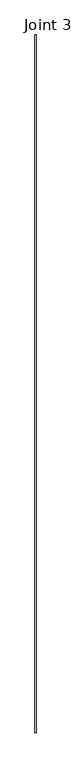
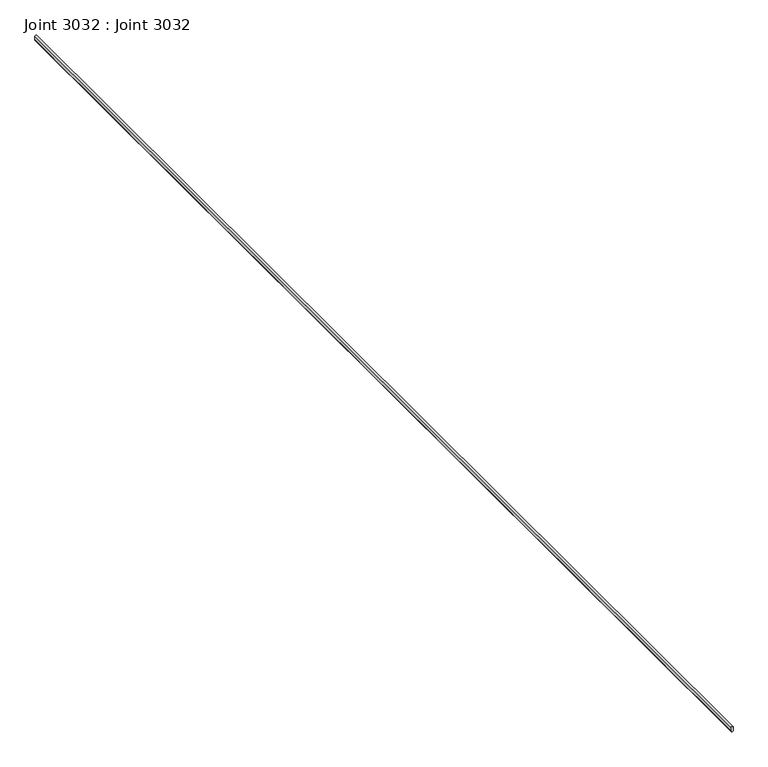
"""IFC4 building model written with IfcOpenShell, lengths in millimetres: proxy geometry, Joint 3032 : Joint 3032."""

from ifc_helpers import new_model, si_unit, point, frame, frame_2d, origin, place, context, project, spatial, polyline, circle_curve, trimmed, segment, composite_curve, outline, extrude, source, transform, mapped, element, save


def joint_3032_joint_3032_122c0fad(model_context):
    return source(origin(), model_context, "Body", "SweptSolid", [
        extrude(outline(composite_curve([segment(polyline([(40328.7531984, -978.1156003), (40334.7081544, -978.1156003)]), True, "CONTINUOUS"), segment(trimmed(circle_curve(frame_2d((40334.7081544, -979.7015378)), 1.5859375), [point((40334.7081544, -978.1156003))], [point((40334.7081544, -981.2874753))], False, "CARTESIAN"), True, "CONTINUOUS"), segment(polyline([(40334.7081544, -981.2874753), (40328.7531984, -981.2874753)]), True, "CONTINUOUS"), segment(trimmed(circle_curve(frame_2d((40328.7531984, -979.7015378)), 1.5859375), [point((40328.7531984, -981.2874753))], [point((40328.7531984, -978.1156003))], False, "CARTESIAN"), True, "CONTINUOUS")], self_intersect=False)), frame((0.0, -1052.8906574, 0.0), z_axis=(0.0, 1.0, 0.0), x_axis=(0.0, 0.0, 1.0)), (0.0, 0.0, 1.0), 2000.0),
    ])


if __name__ == "__main__":
    model = new_model("IFC4")
    model_context = context("Model", 3, world=origin())
    ifc_project = project(units=[si_unit("LENGTHUNIT", "METRE", prefix="MILLI")], contexts=[model_context])
    site = spatial("IfcSite", under=ifc_project)
    building = spatial("IfcBuilding", under=site)
    placement = place(None, origin())
    joint_3032_joint_3032_shape = joint_3032_joint_3032_122c0fad(model_context)
    element("IfcBuildingElementProxy", 1, Name="Joint 3032 : Joint 3032", ObjectType="Joint 3032 : Joint 3032", at=placement, inside=building, context=model_context, shape_type="MappedRepresentation", body=[
        mapped(joint_3032_joint_3032_shape, transform((0.0, 0.0, 0.0), x_axis=(1.0, 0.0, 0.0), y_axis=(0.0, 1.0, 0.0), z_axis=(0.0, 0.0, 1.0))),
    ])
    save(model, "model.ifc")

# Revit data of these elements
# Type "Joint 3032 : Joint 3032"
#   NameOverride = "Joint"
# Element 1 (IfcBuildingElementProxy, "Joint 3032 : Joint 3032")
#   Materials on its faces: "SEALANT"
# Materials
#   "SEALANT": class "Unassigned", colour RGB 142 225 148, transparency 0
